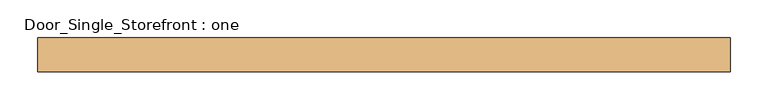
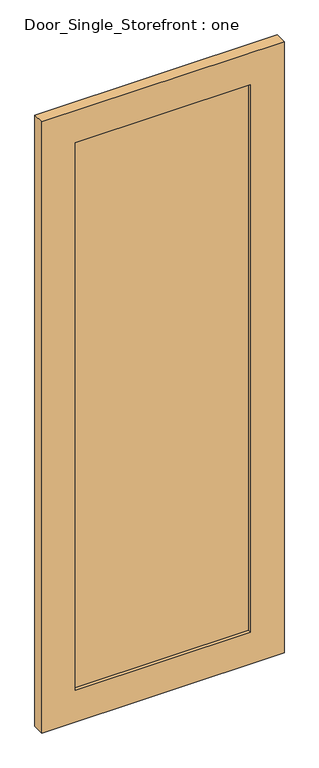
"""IFC4 building model written with IfcOpenShell, lengths in millimetres: door geometry, Door_Single_Storefront : one."""

import ifcopenshell
import ifcopenshell.guid

model = None  # the IFC model being written
_history = None  # IfcOwnerHistory: only IFC2X3 demands one
_inside = {}  # id of a spatial element -> (the spatial element, [elements in it])
_under = {}  # id of a project, library or spatial element -> (it, [spatial elements below it])
_declared = {}  # id of a project -> (the project, [libraries it declares])
_typed = {}  # id of a type object -> (the type object, [elements of that type])
_made_of = {}  # id of a material, layer set ... -> (it, [elements and type objects made of it])


def new_model(schema):
    """Start an empty IFC model of exactly this schema.

    Asked for "IFC4X3", IfcOpenShell would pick the latest addendum, in which some entities
    have other attributes; the version numbers below select the first issue.
    IFC2X3 requires an IfcOwnerHistory on every rooted entity: one is made here for all.
    """
    global model, _history
    if schema == "IFC4X3":
        model = ifcopenshell.file(schema_version=(4, 3, 0, 0))
    else:
        model = ifcopenshell.file(schema=schema)
    _inside.clear()
    _under.clear()
    _declared.clear()
    _typed.clear()
    _made_of.clear()
    _history = None
    if model.schema == "IFC2X3":
        org = make("IfcOrganization", Name="unknown")
        user = make(
            "IfcPersonAndOrganization",
            ThePerson=make("IfcPerson", FamilyName="unknown"),
            TheOrganization=org,
        )
        app = make(
            "IfcApplication",
            ApplicationDeveloper=org,
            Version="unknown",
            ApplicationFullName="unknown",
            ApplicationIdentifier="unknown",
        )
        _history = make(
            "IfcOwnerHistory",
            OwningUser=user,
            OwningApplication=app,
            ChangeAction="ADDED",
            CreationDate=0,
        )
    return model


def make(cls, **values):
    """One entity of the class cls with the attributes given. An attribute that is None is left unset."""
    return model.create_entity(
        cls, **{name: value for name, value in values.items() if value is not None}
    )


def rooted(cls, **values):
    """An entity with a GlobalId (a new one), such as an element, a storey or a relation."""
    return make(cls, GlobalId=ifcopenshell.guid.new(), OwnerHistory=_history, **values)


def si_unit(unit_type, name, prefix=None):
    """IfcSIUnit, for example si_unit("LENGTHUNIT", "METRE", prefix="MILLI")."""
    return make("IfcSIUnit", UnitType=unit_type, Prefix=prefix, Name=name)


def assignment(units):
    """IfcUnitAssignment: the units of a project."""
    return None if units is None else make("IfcUnitAssignment", Units=units)


def point(xyz):
    """IfcCartesianPoint."""
    return None if xyz is None else make("IfcCartesianPoint", Coordinates=xyz)


def direction(xyz):
    """IfcDirection."""
    return None if xyz is None else make("IfcDirection", DirectionRatios=xyz)


def frame(location, z_axis=None, x_axis=None):
    """IfcAxis2Placement3D, a coordinate frame: its origin and axes. An axis left out is left unset."""
    return make(
        "IfcAxis2Placement3D",
        Location=point(location),
        Axis=direction(z_axis),
        RefDirection=direction(x_axis),
    )


def origin():
    """The frame at (0, 0, 0) with its axes left unset."""
    return frame((0.0, 0.0, 0.0))


def place(relative_to, where):
    """IfcLocalPlacement: puts the frame where relative to a parent placement (None: the world)."""
    return make(
        "IfcLocalPlacement", PlacementRelTo=relative_to, RelativePlacement=where
    )


def context(
    kind, dimensions, precision=None, world=None, true_north=None, identifier=None
):
    """IfcGeometricRepresentationContext, for example the 3D "Model" context."""
    return make(
        "IfcGeometricRepresentationContext",
        ContextIdentifier=identifier,
        ContextType=kind,
        CoordinateSpaceDimension=dimensions,
        Precision=precision,
        WorldCoordinateSystem=world,
        TrueNorth=true_north,
    )


def project(units=None, contexts=None):
    """IfcProject with its units and contexts."""
    return rooted(
        "IfcProject",
        Name="project",
        RepresentationContexts=contexts,
        UnitsInContext=assignment(units),
    )


def spatial(cls, under=None, at=None, **own):
    """A site, building, storey or space (cls), placed at a placement, below another one or the project."""
    s = rooted(cls, ObjectPlacement=at, **own)
    if under is not None:
        _under.setdefault(under.id(), (under, []))[1].append(s)
    return s


def polyline(points):
    """IfcPolyline through the points."""
    return make("IfcPolyline", Points=[point(p) for p in points])


def outline(outer, holes=None, kind="AREA"):
    """IfcArbitraryClosedProfileDef: a profile drawn as a closed curve; with holes, ...WithVoids."""
    if holes is None:
        return make("IfcArbitraryClosedProfileDef", ProfileType=kind, OuterCurve=outer)
    return make(
        "IfcArbitraryProfileDefWithVoids",
        ProfileType=kind,
        OuterCurve=outer,
        InnerCurves=holes,
    )


def extrude(swept, where, along, depth):
    """IfcExtrudedAreaSolid: the profile swept, set in the frame where, extruded along a direction by depth."""
    return make(
        "IfcExtrudedAreaSolid",
        SweptArea=swept,
        Position=where,
        ExtrudedDirection=direction(along),
        Depth=depth,
    )


def shape(context_of_items, identifier, shape_type, items):
    """IfcShapeRepresentation: the items that make up one representation, for example the "Body"."""
    return make(
        "IfcShapeRepresentation",
        ContextOfItems=context_of_items,
        RepresentationIdentifier=identifier,
        RepresentationType=shape_type,
        Items=items,
    )


def source(mapping_origin, context_of_items, identifier, shape_type, items):
    """IfcRepresentationMap: a shape defined once, which mapped items show again and again."""
    return make(
        "IfcRepresentationMap",
        MappingOrigin=mapping_origin,
        MappedRepresentation=shape(context_of_items, identifier, shape_type, items),
    )


def transform(
    local_origin,
    x_axis=None,
    y_axis=None,
    z_axis=None,
    scale=None,
    scale2=None,
    scale3=None,
    uniform=True,
):
    """IfcCartesianTransformationOperator3D, or its non-uniform kind. x_axis, y_axis, z_axis: its Axis1, 2, 3."""
    if uniform:
        return make(
            "IfcCartesianTransformationOperator3D",
            Axis1=direction(x_axis),
            Axis2=direction(y_axis),
            LocalOrigin=point(local_origin),
            Scale=scale,
            Axis3=direction(z_axis),
        )
    return make(
        "IfcCartesianTransformationOperator3DnonUniform",
        Axis1=direction(x_axis),
        Axis2=direction(y_axis),
        LocalOrigin=point(local_origin),
        Scale=scale,
        Axis3=direction(z_axis),
        Scale2=scale2,
        Scale3=scale3,
    )


def mapped(mapping_source, mapping_target):
    """IfcMappedItem: shows the shape of a source again, moved by a transform."""
    return make(
        "IfcMappedItem", MappingSource=mapping_source, MappingTarget=mapping_target
    )


def made_of(thing, what):
    """Note that an element or type object is made of a material, layer set ...; save() writes the relation."""
    if what is not None:
        _made_of.setdefault(what.id(), (what, []))[1].append(thing)
    return thing


def element(
    cls,
    number,
    at=None,
    inside=None,
    cuts=None,
    type_object=None,
    material=None,
    context=None,
    identifier="Body",
    shape_type=None,
    held_by="IfcProductDefinitionShape",
    body=None,
    shapes=None,
    **own,
):
    """One element of the class cls, such as IfcWall. Its Tag is "e" and its number.

    at: its placement. inside: the storey or other place that contains it. cuts: it is an
    opening in that element (IfcRelVoidsElement). A single representation is given by context,
    identifier, shape_type and body (its items); several are given by shapes. held_by: the class
    of the entity that holds the representations. save() writes the other relations.
    """
    e = rooted(cls, Tag="e%d" % number, ObjectPlacement=at, **own)
    if body is not None:
        shapes = [shape(context, identifier, shape_type, body)]
    if shapes is not None:
        e.Representation = make(held_by, Representations=shapes)
    if inside is not None:
        _inside.setdefault(inside.id(), (inside, []))[1].append(e)
    if cuts is not None:
        rooted(
            "IfcRelVoidsElement", RelatingBuildingElement=cuts, RelatedOpeningElement=e
        )
    if type_object is not None:
        _typed.setdefault(type_object.id(), (type_object, []))[1].append(e)
    return made_of(e, material)


def aggregate(whole, parts):
    """IfcRelAggregates: a whole, such as a stair, and the parts it consists of."""
    return rooted("IfcRelAggregates", RelatingObject=whole, RelatedObjects=parts)


def save(model, path):
    """Write the relations noted so far, then the file.

    IfcRelAggregates (storeys below a building ...), IfcRelContainedInSpatialStructure (elements
    in a storey), IfcRelDefinesByType, IfcRelAssociatesMaterial and IfcRelDeclares: one each for
    every whole, place, type object, material and project.
    """
    for whole, parts in _under.values():
        aggregate(whole, parts)
    for where, things in _inside.values():
        rooted(
            "IfcRelContainedInSpatialStructure",
            RelatedElements=things,
            RelatingStructure=where,
        )
    for kind, things in _typed.values():
        rooted("IfcRelDefinesByType", RelatedObjects=things, RelatingType=kind)
    for what, things in _made_of.values():
        rooted("IfcRelAssociatesMaterial", RelatedObjects=things, RelatingMaterial=what)
    for by, libraries in _declared.values():
        rooted("IfcRelDeclares", RelatingContext=by, RelatedDefinitions=libraries)
    model.write(path)


def door_single_storefront_one_c51172e4(model_context):
    return source(origin(), model_context, "Body", "SweptSolid", [
        extrude(outline(polyline([(330.2, -6.35), (-330.2, -6.35), (-330.2, 12.7), (330.2, 12.7), (330.2, -6.35)])), frame((0.0, 0.0, 127.0), z_axis=(0.0, 0.0, 1.0), x_axis=(1.0, 0.0, 0.0)), (0.0, 0.0, 1.0), 2184.4),
        extrude(outline(polyline([(2438.4, -457.2), (0.0, -457.2), (0.0, 457.2), (2438.4, 457.2), (2438.4, -457.2)]), holes=[polyline([(127.0, 330.2), (127.0, -330.2), (2311.4, -330.2), (2311.4, 330.2), (127.0, 330.2)])]), frame((0.0, -19.05, 0.0), z_axis=(0.0, 1.0, 0.0), x_axis=(0.0, 0.0, 1.0)), (0.0, 0.0, 1.0), 44.45),
    ])


if __name__ == "__main__":
    model = new_model("IFC4")
    model_context = context("Model", 3, world=origin())
    ifc_project = project(units=[si_unit("LENGTHUNIT", "METRE", prefix="MILLI")], contexts=[model_context])
    site = spatial("IfcSite", under=ifc_project)
    building = spatial("IfcBuilding", under=site)
    placement = place(None, origin())
    door_single_storefront_one_shape = door_single_storefront_one_c51172e4(model_context)
    element("IfcDoor", 1, ObjectType="Door_Single_Storefront : one", at=placement, inside=building, context=model_context, shape_type="MappedRepresentation", body=[
        mapped(door_single_storefront_one_shape, transform((0.0, 0.0, 0.0), x_axis=(1.0, 0.0, 0.0), y_axis=(0.0, 1.0, 0.0), z_axis=(0.0, 0.0, 1.0))),
    ])
    save(model, "model.ifc")

# Revit data of these elements
# Type "Door_Single_Storefront : one"
#   Type Mark = "27"
#   Analytic Construction = "<None>"
#   Stile_Width = 0' - 5"
#   Door_Thickness = 0' - 1 3/4"
#   Door_Offset = 0' - 1"
#   Glass_Material = SAFETY GLAZING
#   Frame_Material = INTERIOR GRADE ALUMINUM STOREFRONT W/ SAFETY GLAZING
#   Function = (empty or 0)
# Element 1 (IfcDoor, "Door_Single_Storefront : one")
#   Materials on its faces: "INTERIOR GRADE ALUMINUM STOREFRONT W/ SAFETY GLAZING", "SAFETY GLAZING"
# Materials
#   "SAFETY GLAZING": class "Glass", colour RGB 142 168 196, transparency 0.75, Description = "Soda Lime Glass", Cost = 0
#   "INTERIOR GRADE ALUMINUM STOREFRONT W/ SAFETY GLAZING": class "Metal", colour RGB 226 226 226, transparency 0, Description = "Aluminum 6061", Cost = 0
